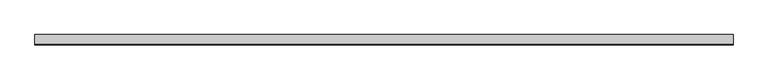
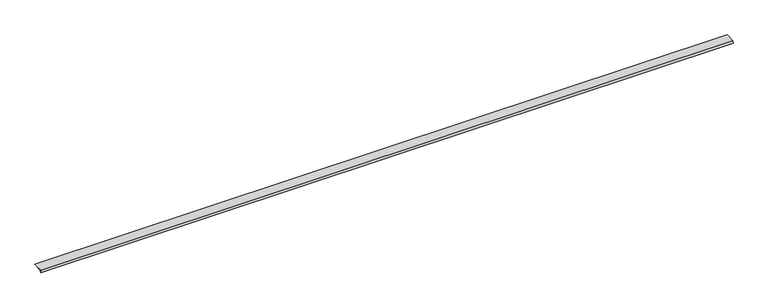
"""IFC4 building model written with IfcOpenShell, lengths in millimetres: proxy geometry, Generic Models 7:Generic Models 1:8:Generic Models 1:8 : Generic Models 7:Generic Models 1:337419:36 : Generic Models 7:Generic Models 1:8:Generic Models 1:8 : Generic Models 7:Generic Models 1:337419:315935."""

import ifcopenshell
import ifcopenshell.guid

model = None  # the IFC model being written
_history = None  # IfcOwnerHistory: only IFC2X3 demands one
_inside = {}  # id of a spatial element -> (the spatial element, [elements in it])
_under = {}  # id of a project, library or spatial element -> (it, [spatial elements below it])
_declared = {}  # id of a project -> (the project, [libraries it declares])
_typed = {}  # id of a type object -> (the type object, [elements of that type])
_made_of = {}  # id of a material, layer set ... -> (it, [elements and type objects made of it])


def new_model(schema):
    """Start an empty IFC model of exactly this schema.

    Asked for "IFC4X3", IfcOpenShell would pick the latest addendum, in which some entities
    have other attributes; the version numbers below select the first issue.
    IFC2X3 requires an IfcOwnerHistory on every rooted entity: one is made here for all.
    """
    global model, _history
    if schema == "IFC4X3":
        model = ifcopenshell.file(schema_version=(4, 3, 0, 0))
    else:
        model = ifcopenshell.file(schema=schema)
    _inside.clear()
    _under.clear()
    _declared.clear()
    _typed.clear()
    _made_of.clear()
    _history = None
    if model.schema == "IFC2X3":
        org = make("IfcOrganization", Name="unknown")
        user = make(
            "IfcPersonAndOrganization",
            ThePerson=make("IfcPerson", FamilyName="unknown"),
            TheOrganization=org,
        )
        app = make(
            "IfcApplication",
            ApplicationDeveloper=org,
            Version="unknown",
            ApplicationFullName="unknown",
            ApplicationIdentifier="unknown",
        )
        _history = make(
            "IfcOwnerHistory",
            OwningUser=user,
            OwningApplication=app,
            ChangeAction="ADDED",
            CreationDate=0,
        )
    return model


def make(cls, **values):
    """One entity of the class cls with the attributes given. An attribute that is None is left unset."""
    return model.create_entity(
        cls, **{name: value for name, value in values.items() if value is not None}
    )


def rooted(cls, **values):
    """An entity with a GlobalId (a new one), such as an element, a storey or a relation."""
    return make(cls, GlobalId=ifcopenshell.guid.new(), OwnerHistory=_history, **values)


def si_unit(unit_type, name, prefix=None):
    """IfcSIUnit, for example si_unit("LENGTHUNIT", "METRE", prefix="MILLI")."""
    return make("IfcSIUnit", UnitType=unit_type, Prefix=prefix, Name=name)


def assignment(units):
    """IfcUnitAssignment: the units of a project."""
    return None if units is None else make("IfcUnitAssignment", Units=units)


def point(xyz):
    """IfcCartesianPoint."""
    return None if xyz is None else make("IfcCartesianPoint", Coordinates=xyz)


def direction(xyz):
    """IfcDirection."""
    return None if xyz is None else make("IfcDirection", DirectionRatios=xyz)


def frame(location, z_axis=None, x_axis=None):
    """IfcAxis2Placement3D, a coordinate frame: its origin and axes. An axis left out is left unset."""
    return make(
        "IfcAxis2Placement3D",
        Location=point(location),
        Axis=direction(z_axis),
        RefDirection=direction(x_axis),
    )


def origin():
    """The frame at (0, 0, 0) with its axes left unset."""
    return frame((0.0, 0.0, 0.0))


def place(relative_to, where):
    """IfcLocalPlacement: puts the frame where relative to a parent placement (None: the world)."""
    return make(
        "IfcLocalPlacement", PlacementRelTo=relative_to, RelativePlacement=where
    )


def context(
    kind, dimensions, precision=None, world=None, true_north=None, identifier=None
):
    """IfcGeometricRepresentationContext, for example the 3D "Model" context."""
    return make(
        "IfcGeometricRepresentationContext",
        ContextIdentifier=identifier,
        ContextType=kind,
        CoordinateSpaceDimension=dimensions,
        Precision=precision,
        WorldCoordinateSystem=world,
        TrueNorth=true_north,
    )


def project(units=None, contexts=None):
    """IfcProject with its units and contexts."""
    return rooted(
        "IfcProject",
        Name="project",
        RepresentationContexts=contexts,
        UnitsInContext=assignment(units),
    )


def spatial(cls, under=None, at=None, **own):
    """A site, building, storey or space (cls), placed at a placement, below another one or the project."""
    s = rooted(cls, ObjectPlacement=at, **own)
    if under is not None:
        _under.setdefault(under.id(), (under, []))[1].append(s)
    return s


def polyline(points):
    """IfcPolyline through the points."""
    return make("IfcPolyline", Points=[point(p) for p in points])


def outline(outer, holes=None, kind="AREA"):
    """IfcArbitraryClosedProfileDef: a profile drawn as a closed curve; with holes, ...WithVoids."""
    if holes is None:
        return make("IfcArbitraryClosedProfileDef", ProfileType=kind, OuterCurve=outer)
    return make(
        "IfcArbitraryProfileDefWithVoids",
        ProfileType=kind,
        OuterCurve=outer,
        InnerCurves=holes,
    )


def extrude(swept, where, along, depth):
    """IfcExtrudedAreaSolid: the profile swept, set in the frame where, extruded along a direction by depth."""
    return make(
        "IfcExtrudedAreaSolid",
        SweptArea=swept,
        Position=where,
        ExtrudedDirection=direction(along),
        Depth=depth,
    )


def shape(context_of_items, identifier, shape_type, items):
    """IfcShapeRepresentation: the items that make up one representation, for example the "Body"."""
    return make(
        "IfcShapeRepresentation",
        ContextOfItems=context_of_items,
        RepresentationIdentifier=identifier,
        RepresentationType=shape_type,
        Items=items,
    )


def source(mapping_origin, context_of_items, identifier, shape_type, items):
    """IfcRepresentationMap: a shape defined once, which mapped items show again and again."""
    return make(
        "IfcRepresentationMap",
        MappingOrigin=mapping_origin,
        MappedRepresentation=shape(context_of_items, identifier, shape_type, items),
    )


def transform(
    local_origin,
    x_axis=None,
    y_axis=None,
    z_axis=None,
    scale=None,
    scale2=None,
    scale3=None,
    uniform=True,
):
    """IfcCartesianTransformationOperator3D, or its non-uniform kind. x_axis, y_axis, z_axis: its Axis1, 2, 3."""
    if uniform:
        return make(
            "IfcCartesianTransformationOperator3D",
            Axis1=direction(x_axis),
            Axis2=direction(y_axis),
            LocalOrigin=point(local_origin),
            Scale=scale,
            Axis3=direction(z_axis),
        )
    return make(
        "IfcCartesianTransformationOperator3DnonUniform",
        Axis1=direction(x_axis),
        Axis2=direction(y_axis),
        LocalOrigin=point(local_origin),
        Scale=scale,
        Axis3=direction(z_axis),
        Scale2=scale2,
        Scale3=scale3,
    )


def mapped(mapping_source, mapping_target):
    """IfcMappedItem: shows the shape of a source again, moved by a transform."""
    return make(
        "IfcMappedItem", MappingSource=mapping_source, MappingTarget=mapping_target
    )


def made_of(thing, what):
    """Note that an element or type object is made of a material, layer set ...; save() writes the relation."""
    if what is not None:
        _made_of.setdefault(what.id(), (what, []))[1].append(thing)
    return thing


def element(
    cls,
    number,
    at=None,
    inside=None,
    cuts=None,
    type_object=None,
    material=None,
    context=None,
    identifier="Body",
    shape_type=None,
    held_by="IfcProductDefinitionShape",
    body=None,
    shapes=None,
    **own,
):
    """One element of the class cls, such as IfcWall. Its Tag is "e" and its number.

    at: its placement. inside: the storey or other place that contains it. cuts: it is an
    opening in that element (IfcRelVoidsElement). A single representation is given by context,
    identifier, shape_type and body (its items); several are given by shapes. held_by: the class
    of the entity that holds the representations. save() writes the other relations.
    """
    e = rooted(cls, Tag="e%d" % number, ObjectPlacement=at, **own)
    if body is not None:
        shapes = [shape(context, identifier, shape_type, body)]
    if shapes is not None:
        e.Representation = make(held_by, Representations=shapes)
    if inside is not None:
        _inside.setdefault(inside.id(), (inside, []))[1].append(e)
    if cuts is not None:
        rooted(
            "IfcRelVoidsElement", RelatingBuildingElement=cuts, RelatedOpeningElement=e
        )
    if type_object is not None:
        _typed.setdefault(type_object.id(), (type_object, []))[1].append(e)
    return made_of(e, material)


def aggregate(whole, parts):
    """IfcRelAggregates: a whole, such as a stair, and the parts it consists of."""
    return rooted("IfcRelAggregates", RelatingObject=whole, RelatedObjects=parts)


def save(model, path):
    """Write the relations noted so far, then the file.

    IfcRelAggregates (storeys below a building ...), IfcRelContainedInSpatialStructure (elements
    in a storey), IfcRelDefinesByType, IfcRelAssociatesMaterial and IfcRelDeclares: one each for
    every whole, place, type object, material and project.
    """
    for whole, parts in _under.values():
        aggregate(whole, parts)
    for where, things in _inside.values():
        rooted(
            "IfcRelContainedInSpatialStructure",
            RelatedElements=things,
            RelatingStructure=where,
        )
    for kind, things in _typed.values():
        rooted("IfcRelDefinesByType", RelatedObjects=things, RelatingType=kind)
    for what, things in _made_of.values():
        rooted("IfcRelAssociatesMaterial", RelatedObjects=things, RelatingMaterial=what)
    for by, libraries in _declared.values():
        rooted("IfcRelDeclares", RelatingContext=by, RelatedDefinitions=libraries)
    model.write(path)


def generic_models_d2b06793(model_context):
    return source(origin(), model_context, "Body", "SweptSolid", [
        extrude(outline(polyline([(-568257.2419692, 8553.2430006), (-568259.0902639, 8553.7729906), (-568254.4589153, 8569.9244227), (-568185.2526825, 8572.8080158), (-568185.1726361, 8570.8869027), (-568252.9929602, 8568.0610559), (-568257.2419692, 8553.2430006)])), frame((591306.0367239, 0.0, 0.0), z_axis=(1.0, 0.0, 0.0), x_axis=(0.0, 1.0, 0.0)), (0.0, 0.0, 1.0), 4876.8),
    ])


if __name__ == "__main__":
    model = new_model("IFC4")
    model_context = context("Model", 3, world=origin())
    ifc_project = project(units=[si_unit("LENGTHUNIT", "METRE", prefix="MILLI")], contexts=[model_context])
    site = spatial("IfcSite", under=ifc_project)
    building = spatial("IfcBuilding", under=site)
    placement = place(None, origin())
    generic_models_shape = generic_models_d2b06793(model_context)
    element("IfcBuildingElementProxy", 1, Name="Generic Models 7:Generic Models 1:8:Generic Models 1:8 : Generic Models 7:Generic Models 1:337419:36 : Generic Models 7:Generic Models 1:8:Generic Models 1:8 : Generic Models 7:Generic Models 1:337419:315935", ObjectType="Generic Models 7:Generic Models 1:8:Generic Models 1:8 : Generic Models 7:Generic Models 1:337419:36 : Generic Models 7:Generic Models 1:8:Generic Models 1:8 : Generic Models 7:Generic Models 1:337419:315935", at=placement, inside=building, context=model_context, shape_type="MappedRepresentation", body=[
        mapped(generic_models_shape, transform((0.0, 0.0, 0.0), x_axis=(1.0, 0.0, 0.0), y_axis=(0.0, 1.0, 0.0), z_axis=(0.0, 0.0, 1.0))),
    ])
    save(model, "model.ifc")

# Revit data of these elements
# Type "Generic Models 7:Generic Models 1:8:Generic Models 1:8 : Generic Models 7:Generic Models 1:337419:36 : Generic Models 7:Generic Models 1:8:Generic Models 1:8 : Generic Models 7:Generic Models 1:337419:315935"
#   NameOverride = "Generic Models 7:Generic Models 1:8:Generic Models 1:8 : Generic Models 7:Generic Models 1:337419:315935"
#   ObjectTypeOverride = "Generic Models 1:8 : Generic Models 7:Generic Models 1:337419"
#   Reference = "Generic Models 1"
#   Tag = "315935"
# Element 1 (IfcBuildingElementProxy, "Generic Models 7:Generic Models 1:8:Generic Models 1:8 : Generic Models 7:Generic Models 1:337419:36 : Generic Models 7:Generic Models 1:8:Generic Models 1:8 : Generic Models 7:Generic Models 1:337419:315935")
#   Materials on its faces: "DRIP EDGE FLASHING"
# Materials
#   "DRIP EDGE FLASHING": class "Unassigned", colour RGB 210 209 208, transparency 0, Cost = 0
